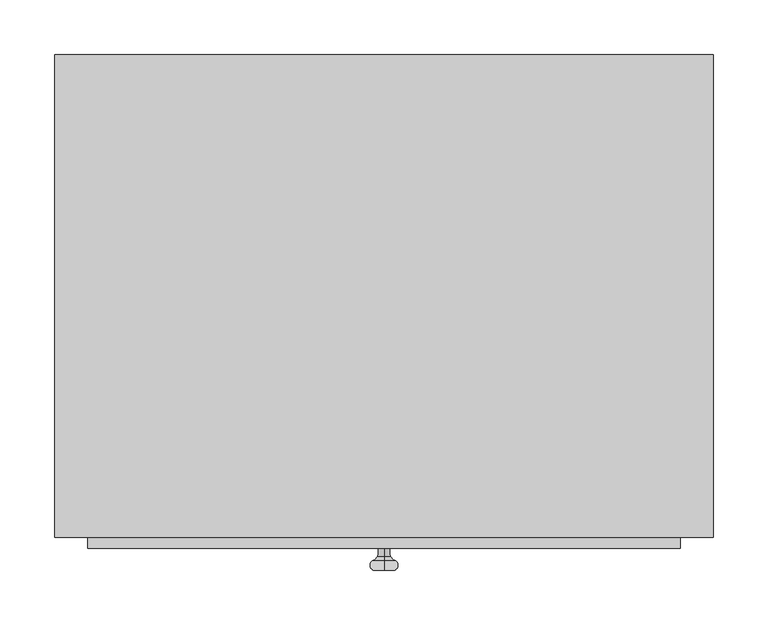
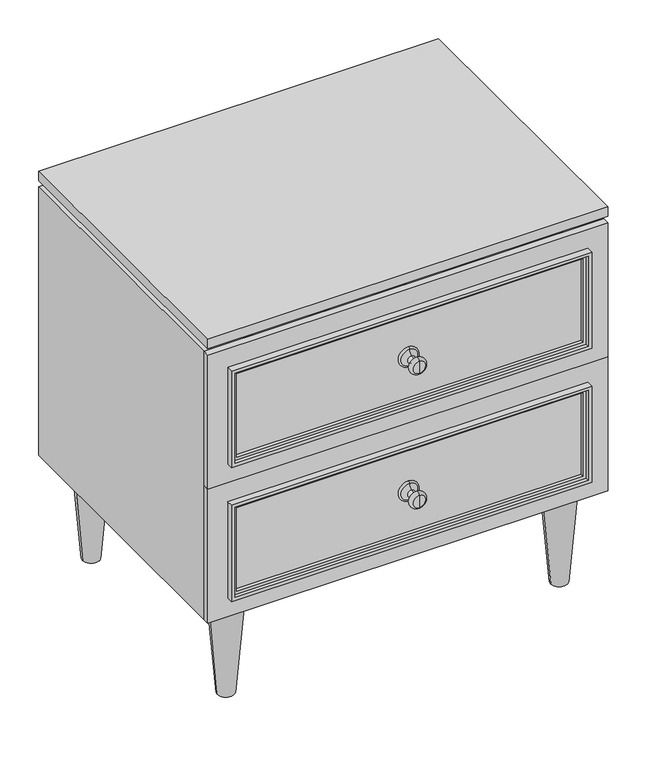
"""IFC4 building model written with IfcOpenShell, lengths in millimetres: proxy geometry, Criado Mudo 02 : Criado Mudo 02."""

from ifc_helpers import new_model, si_unit, point, frame, origin, place, context, project, spatial, polyline, circle_curve, ellipse_curve, trimmed, outline, extrude, faceted_brep, source, transform, mapped, element, save
from ifc_brep_helpers import plane_surface, revolved_surface, advanced_brep


def generic_models_2b41c82f(model_context):
    return source(origin(), model_context, "Body", "SolidModel", [
        advanced_brep(
        [(-237.3303343, 175.0, 0.0), (-262.6696657, 175.0, 0.0), (-225.0, 175.0, 150.0), (-275.0, 175.0, 150.0)],
        [
            (0, 1, circle_curve(frame((-250.0, 175.0, 0.0), z_axis=(0.0, 0.0, -1.0), x_axis=(-1.0, 0.0, 0.0)), 12.6696657)),
            (1, 0, circle_curve(frame((-250.0, 175.0, 0.0), z_axis=(0.0, 0.0, -1.0), x_axis=(1.0, 0.0, 0.0)), 12.6696657)),
            (2, 3, circle_curve(frame((-250.0, 175.0, 150.0), z_axis=(0.0, 0.0, 1.0), x_axis=(1.0, 0.0, 0.0)), 25.0)),
            (3, 2, circle_curve(frame((-250.0, 175.0, 150.0), z_axis=(0.0, 0.0, 1.0), x_axis=(-1.0, 0.0, 0.0)), 25.0)),
            (2, 0),
            (1, 3),
        ],
        [
            plane_surface(frame((-250.0, 175.0, 0.0), z_axis=(0.0, 0.0, -1.0), x_axis=(0.0, -1.0, 0.0))),
            plane_surface(frame((-250.0, 175.0, 150.0), z_axis=(0.0, 0.0, 1.0), x_axis=(0.0, -1.0, 0.0))),
            revolved_surface(polyline([(-237.33033426755935, 175.0, 0.0), (-225.0, 175.0, 150.0)]), (-250.0, 175.0, -154.1280081), (0.0, 0.0, 1.0)),
            revolved_surface(polyline([(-262.66966573244065, 175.0, 0.0), (-275.0, 175.0, 150.0)]), (-250.0, 175.0, -154.1280081), (0.0, 0.0, 1.0)),
        ],
        [
            (0, [[1, 2]]),
            (1, [[3, 4]]),
            (2, [[5, -2, 6, -3]]),
            (3, [[-6, -1, -5, -4]]),
        ],
    ),
        advanced_brep(
        [(237.3303343, 175.0, 0.0), (262.6696657, 175.0, 0.0), (225.0, 175.0, 150.0), (275.0, 175.0, 150.0)],
        [
            (0, 1, circle_curve(frame((250.0, 175.0, 0.0), z_axis=(0.0, 0.0, -1.0), x_axis=(-1.0, 0.0, 0.0)), 12.6696657)),
            (1, 0, circle_curve(frame((250.0, 175.0, 0.0), z_axis=(0.0, 0.0, -1.0), x_axis=(1.0, 0.0, 0.0)), 12.6696657)),
            (2, 3, circle_curve(frame((250.0, 175.0, 150.0), z_axis=(0.0, 0.0, 1.0), x_axis=(1.0, 0.0, 0.0)), 25.0)),
            (3, 2, circle_curve(frame((250.0, 175.0, 150.0), z_axis=(0.0, 0.0, 1.0), x_axis=(-1.0, 0.0, 0.0)), 25.0)),
            (3, 1),
            (0, 2),
        ],
        [
            plane_surface(frame((250.0, 175.0, 0.0), z_axis=(0.0, 0.0, -1.0), x_axis=(0.0, -1.0, 0.0))),
            plane_surface(frame((250.0, 175.0, 150.0), z_axis=(0.0, 0.0, 1.0), x_axis=(0.0, -1.0, 0.0))),
            revolved_surface(polyline([(237.33033426755935, 175.0, 0.0), (225.0, 175.0, 150.0)]), (250.0, 175.0, -154.1280081), (0.0, 0.0, 1.0)),
            revolved_surface(polyline([(262.66966573244065, 175.0, 0.0), (275.0, 175.0, 150.0)]), (250.0, 175.0, -154.1280081), (0.0, 0.0, 1.0)),
        ],
        [
            (0, [[1, 2]]),
            (1, [[3, 4]]),
            (2, [[-4, 5, -1, 6]]),
            (3, [[-3, -6, -2, -5]]),
        ],
    ),
        advanced_brep(
        [(237.3303343, -175.0, 0.0), (262.6696657, -175.0, 0.0), (225.0, -175.0, 150.0), (275.0, -175.0, 150.0)],
        [
            (0, 1, circle_curve(frame((250.0, -175.0, 0.0), z_axis=(0.0, 0.0, -1.0), x_axis=(1.0, 0.0, 0.0)), 12.6696657)),
            (1, 0, circle_curve(frame((250.0, -175.0, 0.0), z_axis=(0.0, 0.0, -1.0), x_axis=(-1.0, 0.0, 0.0)), 12.6696657)),
            (2, 3, circle_curve(frame((250.0, -175.0, 150.0), z_axis=(0.0, 0.0, 1.0), x_axis=(-1.0, 0.0, 0.0)), 25.0)),
            (3, 2, circle_curve(frame((250.0, -175.0, 150.0), z_axis=(0.0, 0.0, 1.0), x_axis=(1.0, 0.0, 0.0)), 25.0)),
            (2, 0),
            (1, 3),
        ],
        [
            plane_surface(frame((250.0, -175.0, 0.0), z_axis=(0.0, 0.0, -1.0), x_axis=(0.0, 1.0, 0.0))),
            plane_surface(frame((250.0, -175.0, 150.0), z_axis=(0.0, 0.0, 1.0), x_axis=(0.0, 1.0, 0.0))),
            revolved_surface(polyline([(237.33033426755935, -175.0, 0.0), (225.0, -175.0, 150.0)]), (250.0, -175.0, -154.1280081), (0.0, 0.0, 1.0)),
            revolved_surface(polyline([(262.66966573244065, -175.0, 0.0), (275.0, -175.0, 150.0)]), (250.0, -175.0, -154.1280081), (0.0, 0.0, 1.0)),
        ],
        [
            (0, [[1, 2]]),
            (1, [[3, 4]]),
            (2, [[5, -2, 6, -3]]),
            (3, [[-6, -1, -5, -4]]),
        ],
    ),
        advanced_brep(
        [(-237.3303343, -175.0, 0.0), (-262.6696657, -175.0, 0.0), (-225.0, -175.0, 150.0), (-275.0, -175.0, 150.0)],
        [
            (0, 1, circle_curve(frame((-250.0, -175.0, 0.0), z_axis=(0.0, 0.0, -1.0), x_axis=(1.0, 0.0, 0.0)), 12.6696657)),
            (1, 0, circle_curve(frame((-250.0, -175.0, 0.0), z_axis=(0.0, 0.0, -1.0), x_axis=(-1.0, 0.0, 0.0)), 12.6696657)),
            (2, 3, circle_curve(frame((-250.0, -175.0, 150.0), z_axis=(0.0, 0.0, 1.0), x_axis=(-1.0, 0.0, 0.0)), 25.0)),
            (3, 2, circle_curve(frame((-250.0, -175.0, 150.0), z_axis=(0.0, 0.0, 1.0), x_axis=(1.0, 0.0, 0.0)), 25.0)),
            (3, 1),
            (0, 2),
        ],
        [
            plane_surface(frame((-250.0, -175.0, 0.0), z_axis=(0.0, 0.0, -1.0), x_axis=(0.0, 1.0, 0.0))),
            plane_surface(frame((-250.0, -175.0, 150.0), z_axis=(0.0, 0.0, 1.0), x_axis=(0.0, 1.0, 0.0))),
            revolved_surface(polyline([(-237.33033426755935, -175.0, 0.0), (-225.0, -175.0, 150.0)]), (-250.0, -175.0, -154.1280081), (0.0, 0.0, 1.0)),
            revolved_surface(polyline([(-262.66966573244065, -175.0, 0.0), (-275.0, -175.0, 150.0)]), (-250.0, -175.0, -154.1280081), (0.0, 0.0, 1.0)),
        ],
        [
            (0, [[1, 2]]),
            (1, [[3, 4]]),
            (2, [[-4, 5, -1, 6]]),
            (3, [[-3, -6, -2, -5]]),
        ],
    ),
        advanced_brep(
        [(0.0, -219.1088234, 455.5505414), (0.0, -219.1088234, 481.9494586), (0.0, -215.0, 481.9494586), (0.0, -215.0, 455.5505414), (0.0, -224.0337931, 462.8521094), (0.0, -224.0337931, 474.6478906), (0.0, -232.2529022, 462.8521094), (0.0, -232.2529022, 474.6478906), (0.0, -236.1458139, 458.9591976), (0.0, -236.1458139, 478.5408024), (0.0, -245.0, 458.9591976), (0.0, -245.0, 478.5408024), (0.0, -245.0, 468.75), (0.0, -215.0, 468.75)],
        [
            (0, 1, circle_curve(frame((0.0, -219.1088234, 468.75), z_axis=(0.0, 1.0, 0.0), x_axis=(0.0, 0.0, 1.0)), 13.1994586)),
            (1, 2, circle_curve(frame((0.0, -217.0544117, 481.9494586), z_axis=(-1.0, 0.0, 0.0), x_axis=(0.0, -1.0, 0.0)), 2.0544117)),
            (2, 3, circle_curve(frame((0.0, -215.0, 468.75), z_axis=(0.0, -1.0, 0.0), x_axis=(0.0, 0.0, 1.0)), 13.1994586)),
            (3, 0, circle_curve(frame((0.0, -217.0544117, 455.5505414), z_axis=(-1.0, 0.0, 0.0), x_axis=(0.0, -1.0, 0.0)), 2.0544117)),
            (1, 0, circle_curve(frame((0.0, -219.1088234, 468.75), z_axis=(0.0, 1.0, 0.0), x_axis=(0.0, 0.0, 1.0)), 13.1994586)),
            (3, 2, circle_curve(frame((0.0, -215.0, 468.75), z_axis=(0.0, -1.0, 0.0), x_axis=(0.0, 0.0, 1.0)), 13.1994586)),
            (4, 5, circle_curve(frame((0.0, -224.0337931, 468.75), z_axis=(0.0, 1.0, 0.0), x_axis=(0.0, 0.0, 1.0)), 5.8978906)),
            (5, 1, circle_curve(frame((0.0, -226.9838181, 481.9494586), z_axis=(1.0, 0.0, 0.0), x_axis=(0.0, -1.0, 0.0)), 7.8749947)),
            (0, 4, circle_curve(frame((0.0, -226.9838181, 455.5505414), z_axis=(1.0, 0.0, 0.0), x_axis=(0.0, -1.0, 0.0)), 7.8749947)),
            (5, 4, circle_curve(frame((0.0, -224.0337931, 468.75), z_axis=(0.0, 1.0, 0.0), x_axis=(0.0, 0.0, 1.0)), 5.8978906)),
            (6, 7, circle_curve(frame((0.0, -232.2529022, 468.75), z_axis=(0.0, 1.0, 0.0), x_axis=(0.0, 0.0, 1.0)), 5.8978906)),
            (7, 5, circle_curve(frame((0.0, -228.1433476, 484.819395), z_axis=(1.0, 0.0, 0.0), x_axis=(0.0, -1.0, 0.0)), 10.9703208)),
            (4, 6, circle_curve(frame((0.0, -228.1433476, 452.680605), z_axis=(1.0, 0.0, 0.0), x_axis=(0.0, -1.0, 0.0)), 10.9703208)),
            (7, 6, circle_curve(frame((0.0, -232.2529022, 468.75), z_axis=(0.0, 1.0, 0.0), x_axis=(0.0, 0.0, 1.0)), 5.8978906)),
            (8, 9, circle_curve(frame((0.0, -236.1458139, 468.75), z_axis=(0.0, 1.0, 0.0), x_axis=(0.0, 0.0, 1.0)), 9.7908024)),
            (9, 7, circle_curve(frame((0.0, -229.6137954, 481.1799091), z_axis=(1.0, 0.0, 0.0), x_axis=(0.0, -1.0, 0.0)), 7.0450089)),
            (6, 8, circle_curve(frame((0.0, -229.6137954, 456.3200909), z_axis=(1.0, 0.0, 0.0), x_axis=(0.0, -1.0, 0.0)), 7.0450089)),
            (9, 8, circle_curve(frame((0.0, -236.1458139, 468.75), z_axis=(0.0, 1.0, 0.0), x_axis=(0.0, 0.0, 1.0)), 9.7908024)),
            (10, 11, circle_curve(frame((0.0, -245.0, 468.75), z_axis=(0.0, 1.0, 0.0), x_axis=(0.0, 0.0, 1.0)), 9.7908024)),
            (11, 9, circle_curve(frame((0.0, -240.5729069, 476.7521407), z_axis=(-1.0, 0.0, 0.0), x_axis=(0.0, -1.0, 0.0)), 4.7747737)),
            (8, 10, circle_curve(frame((0.0, -240.5729069, 460.7478593), z_axis=(-1.0, 0.0, 0.0), x_axis=(0.0, -1.0, 0.0)), 4.7747737)),
            (11, 10, circle_curve(frame((0.0, -245.0, 468.75), z_axis=(0.0, 1.0, 0.0), x_axis=(0.0, 0.0, 1.0)), 9.7908024)),
            (12, 11),
            (10, 12),
            (2, 13),
            (13, 3),
        ],
        [
            revolved_surface(trimmed(ellipse_curve(frame((0.0, -217.0544117, 481.9494586), z_axis=(1.0, 0.0, 0.0), x_axis=(0.0, -1.0, 0.0)), 2.0544117, 2.0544117), [point((0.0, -215.0, 481.9494586))], [point((0.0, -219.1088234, 481.9494586))], True, "CARTESIAN"), (0.0, -215.0, 468.75), (0.0, -1.0, 0.0)),
            revolved_surface(trimmed(ellipse_curve(frame((0.0, -226.9838181, 481.9494586), z_axis=(-1.0, 0.0, 0.0), x_axis=(0.0, -1.0, 0.0)), 7.8749947, 7.8749947), [point((0.0, -219.1088234, 481.9494586))], [point((0.0, -224.0337931, 474.6478906))], True, "CARTESIAN"), (0.0, -215.0, 468.75), (0.0, -1.0, 0.0)),
            revolved_surface(trimmed(ellipse_curve(frame((0.0, -228.1433476, 484.819395), z_axis=(-1.0, 0.0, 0.0), x_axis=(0.0, -1.0, 0.0)), 10.9703208, 10.9703208), [point((0.0, -224.0337931, 474.6478906))], [point((0.0, -232.2529022, 474.6478906))], True, "CARTESIAN"), (0.0, -215.0, 468.75), (0.0, -1.0, 0.0)),
            revolved_surface(trimmed(ellipse_curve(frame((0.0, -229.6137954, 481.1799091), z_axis=(-1.0, 0.0, 0.0), x_axis=(0.0, -1.0, 0.0)), 7.0450089, 7.0450089), [point((0.0, -232.2529022, 474.6478906))], [point((0.0, -236.1458139, 478.5408024))], True, "CARTESIAN"), (0.0, -215.0, 468.75), (0.0, -1.0, 0.0)),
            revolved_surface(trimmed(ellipse_curve(frame((0.0, -240.5729069, 476.7521407), z_axis=(1.0, 0.0, 0.0), x_axis=(0.0, -1.0, 0.0)), 4.7747737, 4.7747737), [point((0.0, -236.1458139, 478.5408024))], [point((0.0, -245.0, 478.5408024))], True, "CARTESIAN"), (0.0, -215.0, 468.75), (0.0, -1.0, 0.0)),
            plane_surface(frame((0.0, -245.0, 468.75), z_axis=(0.0, -1.0, 0.0), x_axis=(0.0, 0.0, 1.0))),
            plane_surface(frame((0.0, -215.0, 468.75), z_axis=(0.0, 1.0, 0.0), x_axis=(0.0, 0.0, 1.0))),
        ],
        [
            (0, [[1, 2, 3, 4]]),
            (0, [[5, -4, 6, -2]]),
            (1, [[7, 8, -1, 9]]),
            (1, [[10, -9, -5, -8]]),
            (2, [[11, 12, -7, 13]]),
            (2, [[14, -13, -10, -12]]),
            (3, [[15, 16, -11, 17]]),
            (3, [[18, -17, -14, -16]]),
            (4, [[19, 20, -15, 21]]),
            (4, [[22, -21, -18, -20]]),
            (5, [[23, -19, 24]]),
            (5, [[-24, -22, -23]]),
            (6, [[-3, 25, 26]]),
            (6, [[-6, -26, -25]]),
        ],
    ),
        faceted_brep([(270.0, -215.0, 545.0), (270.0, -225.0, 545.0), (270.0, -225.0, 392.5), (270.0, -215.0, 392.5), (260.0, -220.0, 535.0), (260.0, -215.0, 535.0), (260.0, -215.0, 402.5), (260.0, -220.0, 402.5), (265.0, -225.0, 540.0), (265.0, -220.0, 540.0), (265.0, -220.0, 397.5), (265.0, -225.0, 397.5), (-270.0, -225.0, 392.5), (-270.0, -215.0, 392.5), (-260.0, -215.0, 402.5), (-260.0, -220.0, 402.5), (-265.0, -220.0, 397.5), (-265.0, -225.0, 397.5), (-270.0, -225.0, 545.0), (-270.0, -215.0, 545.0), (-260.0, -215.0, 535.0), (-260.0, -220.0, 535.0), (-265.0, -220.0, 540.0), (-265.0, -225.0, 540.0)], [[[0, 1, 2, 3]], [[4, 5, 6, 7]], [[8, 9, 10, 11]], [[3, 2, 12, 13]], [[7, 6, 14, 15]], [[11, 10, 16, 17]], [[13, 12, 18, 19]], [[15, 14, 20, 21]], [[17, 16, 22, 23]], [[19, 18, 1, 0]], [[3, 13, 19, 0], [5, 20, 14, 6]], [[21, 20, 5, 4]], [[9, 22, 16, 10], [7, 15, 21, 4]], [[23, 22, 9, 8]], [[1, 18, 12, 2], [11, 17, 23, 8]]]),
        extrude(outline(polyline([(300.0, -215.0), (-300.0, -215.0), (-300.0, -205.0), (300.0, -205.0), (300.0, -215.0)])), frame((0.0, 0.0, 362.5), z_axis=(0.0, 0.0, 1.0), x_axis=(1.0, 0.0, 0.0)), (0.0, 0.0, 1.0), 212.5),
        extrude(outline(polyline([(277.5, -205.0), (-277.5, -205.0), (-277.5, 200.0), (277.5, 200.0), (277.5, -205.0)])), frame((0.0, 0.0, 392.5), z_axis=(0.0, 0.0, 1.0), x_axis=(1.0, 0.0, 0.0)), (0.0, 0.0, 1.0), 15.0),
        extrude(outline(polyline([(262.5, 200.0), (262.5, 185.0), (-262.5, 185.0), (-262.5, 200.0), (262.5, 200.0)])), frame((0.0, 0.0, 407.5), z_axis=(0.0, 0.0, 1.0), x_axis=(1.0, 0.0, 0.0)), (0.0, 0.0, 1.0), 137.5),
        extrude(outline(polyline([(262.5, 200.0), (277.5, 200.0), (277.5, -205.0), (262.5, -205.0), (262.5, 200.0)])), frame((0.0, 0.0, 407.5), z_axis=(0.0, 0.0, 1.0), x_axis=(1.0, 0.0, 0.0)), (0.0, 0.0, 1.0), 137.5),
        extrude(outline(polyline([(-262.5, 200.0), (-262.5, -205.0), (-277.5, -205.0), (-277.5, 200.0), (-262.5, 200.0)])), frame((0.0, 0.0, 407.5), z_axis=(0.0, 0.0, 1.0), x_axis=(1.0, 0.0, 0.0)), (0.0, 0.0, 1.0), 137.5),
        advanced_brep(
        [(0.0, -219.1088234, 243.0505414), (0.0, -219.1088234, 269.4494586), (0.0, -215.0, 269.4494586), (0.0, -215.0, 243.0505414), (0.0, -224.0337931, 250.3521094), (0.0, -224.0337931, 262.1478906), (0.0, -232.2529022, 250.3521094), (0.0, -232.2529022, 262.1478906), (0.0, -236.1458139, 246.4591976), (0.0, -236.1458139, 266.0408024), (0.0, -245.0, 246.4591976), (0.0, -245.0, 266.0408024), (0.0, -245.0, 256.25), (0.0, -215.0, 256.25)],
        [
            (0, 1, circle_curve(frame((0.0, -219.1088234, 256.25), z_axis=(0.0, 1.0, 0.0), x_axis=(0.0, 0.0, 1.0)), 13.1994586)),
            (1, 2, circle_curve(frame((0.0, -217.0544117, 269.4494586), z_axis=(-1.0, 0.0, 0.0), x_axis=(0.0, -1.0, 0.0)), 2.0544117)),
            (2, 3, circle_curve(frame((0.0, -215.0, 256.25), z_axis=(0.0, -1.0, 0.0), x_axis=(0.0, 0.0, 1.0)), 13.1994586)),
            (3, 0, circle_curve(frame((0.0, -217.0544117, 243.0505414), z_axis=(-1.0, 0.0, 0.0), x_axis=(0.0, -1.0, 0.0)), 2.0544117)),
            (1, 0, circle_curve(frame((0.0, -219.1088234, 256.25), z_axis=(0.0, 1.0, 0.0), x_axis=(0.0, 0.0, 1.0)), 13.1994586)),
            (3, 2, circle_curve(frame((0.0, -215.0, 256.25), z_axis=(0.0, -1.0, 0.0), x_axis=(0.0, 0.0, 1.0)), 13.1994586)),
            (4, 5, circle_curve(frame((0.0, -224.0337931, 256.25), z_axis=(0.0, 1.0, 0.0), x_axis=(0.0, 0.0, 1.0)), 5.8978906)),
            (5, 1, circle_curve(frame((0.0, -226.9838181, 269.4494586), z_axis=(1.0, 0.0, 0.0), x_axis=(0.0, -1.0, 0.0)), 7.8749947)),
            (0, 4, circle_curve(frame((0.0, -226.9838181, 243.0505414), z_axis=(1.0, 0.0, 0.0), x_axis=(0.0, -1.0, 0.0)), 7.8749947)),
            (5, 4, circle_curve(frame((0.0, -224.0337931, 256.25), z_axis=(0.0, 1.0, 0.0), x_axis=(0.0, 0.0, 1.0)), 5.8978906)),
            (6, 7, circle_curve(frame((0.0, -232.2529022, 256.25), z_axis=(0.0, 1.0, 0.0), x_axis=(0.0, 0.0, 1.0)), 5.8978906)),
            (7, 5, circle_curve(frame((0.0, -228.1433476, 272.319395), z_axis=(1.0, 0.0, 0.0), x_axis=(0.0, -1.0, 0.0)), 10.9703208)),
            (4, 6, circle_curve(frame((0.0, -228.1433476, 240.180605), z_axis=(1.0, 0.0, 0.0), x_axis=(0.0, -1.0, 0.0)), 10.9703208)),
            (7, 6, circle_curve(frame((0.0, -232.2529022, 256.25), z_axis=(0.0, 1.0, 0.0), x_axis=(0.0, 0.0, 1.0)), 5.8978906)),
            (8, 9, circle_curve(frame((0.0, -236.1458139, 256.25), z_axis=(0.0, 1.0, 0.0), x_axis=(0.0, 0.0, 1.0)), 9.7908024)),
            (9, 7, circle_curve(frame((0.0, -229.6137954, 268.6799091), z_axis=(1.0, 0.0, 0.0), x_axis=(0.0, -1.0, 0.0)), 7.0450089)),
            (6, 8, circle_curve(frame((0.0, -229.6137954, 243.8200909), z_axis=(1.0, 0.0, 0.0), x_axis=(0.0, -1.0, 0.0)), 7.0450089)),
            (9, 8, circle_curve(frame((0.0, -236.1458139, 256.25), z_axis=(0.0, 1.0, 0.0), x_axis=(0.0, 0.0, 1.0)), 9.7908024)),
            (10, 11, circle_curve(frame((0.0, -245.0, 256.25), z_axis=(0.0, 1.0, 0.0), x_axis=(0.0, 0.0, 1.0)), 9.7908024)),
            (11, 9, circle_curve(frame((0.0, -240.5729069, 264.2521407), z_axis=(-1.0, 0.0, 0.0), x_axis=(0.0, -1.0, 0.0)), 4.7747737)),
            (8, 10, circle_curve(frame((0.0, -240.5729069, 248.2478593), z_axis=(-1.0, 0.0, 0.0), x_axis=(0.0, -1.0, 0.0)), 4.7747737)),
            (11, 10, circle_curve(frame((0.0, -245.0, 256.25), z_axis=(0.0, 1.0, 0.0), x_axis=(0.0, 0.0, 1.0)), 9.7908024)),
            (12, 11),
            (10, 12),
            (2, 13),
            (13, 3),
        ],
        [
            revolved_surface(trimmed(ellipse_curve(frame((0.0, -217.0544117, 269.4494586), z_axis=(1.0, 0.0, 0.0), x_axis=(0.0, -1.0, 0.0)), 2.0544117, 2.0544117), [point((0.0, -215.0, 269.4494586))], [point((0.0, -219.1088234, 269.4494586))], True, "CARTESIAN"), (0.0, -215.0, 256.25), (0.0, -1.0, 0.0)),
            revolved_surface(trimmed(ellipse_curve(frame((0.0, -226.9838181, 269.4494586), z_axis=(-1.0, 0.0, 0.0), x_axis=(0.0, -1.0, 0.0)), 7.8749947, 7.8749947), [point((0.0, -219.1088234, 269.4494586))], [point((0.0, -224.0337931, 262.1478906))], True, "CARTESIAN"), (0.0, -215.0, 256.25), (0.0, -1.0, 0.0)),
            revolved_surface(trimmed(ellipse_curve(frame((0.0, -228.1433476, 272.319395), z_axis=(-1.0, 0.0, 0.0), x_axis=(0.0, -1.0, 0.0)), 10.9703208, 10.9703208), [point((0.0, -224.0337931, 262.1478906))], [point((0.0, -232.2529022, 262.1478906))], True, "CARTESIAN"), (0.0, -215.0, 256.25), (0.0, -1.0, 0.0)),
            revolved_surface(trimmed(ellipse_curve(frame((0.0, -229.6137954, 268.6799091), z_axis=(-1.0, 0.0, 0.0), x_axis=(0.0, -1.0, 0.0)), 7.0450089, 7.0450089), [point((0.0, -232.2529022, 262.1478906))], [point((0.0, -236.1458139, 266.0408024))], True, "CARTESIAN"), (0.0, -215.0, 256.25), (0.0, -1.0, 0.0)),
            revolved_surface(trimmed(ellipse_curve(frame((0.0, -240.5729069, 264.2521407), z_axis=(1.0, 0.0, 0.0), x_axis=(0.0, -1.0, 0.0)), 4.7747737, 4.7747737), [point((0.0, -236.1458139, 266.0408024))], [point((0.0, -245.0, 266.0408024))], True, "CARTESIAN"), (0.0, -215.0, 256.25), (0.0, -1.0, 0.0)),
            plane_surface(frame((0.0, -245.0, 256.25), z_axis=(0.0, -1.0, 0.0), x_axis=(0.0, 0.0, 1.0))),
            plane_surface(frame((0.0, -215.0, 256.25), z_axis=(0.0, 1.0, 0.0), x_axis=(0.0, 0.0, 1.0))),
        ],
        [
            (0, [[1, 2, 3, 4]]),
            (0, [[5, -4, 6, -2]]),
            (1, [[7, 8, -1, 9]]),
            (1, [[10, -9, -5, -8]]),
            (2, [[11, 12, -7, 13]]),
            (2, [[14, -13, -10, -12]]),
            (3, [[15, 16, -11, 17]]),
            (3, [[18, -17, -14, -16]]),
            (4, [[19, 20, -15, 21]]),
            (4, [[22, -21, -18, -20]]),
            (5, [[23, -19, 24]]),
            (5, [[-24, -22, -23]]),
            (6, [[-3, 25, 26]]),
            (6, [[-6, -26, -25]]),
        ],
    ),
        faceted_brep([(270.0, -215.0, 332.5), (270.0, -225.0, 332.5), (270.0, -225.0, 180.0), (270.0, -215.0, 180.0), (260.0, -220.0, 322.5), (260.0, -215.0, 322.5), (260.0, -215.0, 190.0), (260.0, -220.0, 190.0), (265.0, -225.0, 327.5), (265.0, -220.0, 327.5), (265.0, -220.0, 185.0), (265.0, -225.0, 185.0), (-270.0, -225.0, 180.0), (-270.0, -215.0, 180.0), (-260.0, -215.0, 190.0), (-260.0, -220.0, 190.0), (-265.0, -220.0, 185.0), (-265.0, -225.0, 185.0), (-270.0, -225.0, 332.5), (-270.0, -215.0, 332.5), (-260.0, -215.0, 322.5), (-260.0, -220.0, 322.5), (-265.0, -220.0, 327.5), (-265.0, -225.0, 327.5)], [[[0, 1, 2, 3]], [[4, 5, 6, 7]], [[8, 9, 10, 11]], [[3, 2, 12, 13]], [[7, 6, 14, 15]], [[11, 10, 16, 17]], [[13, 12, 18, 19]], [[15, 14, 20, 21]], [[17, 16, 22, 23]], [[19, 18, 1, 0]], [[3, 13, 19, 0], [5, 20, 14, 6]], [[21, 20, 5, 4]], [[9, 22, 16, 10], [7, 15, 21, 4]], [[23, 22, 9, 8]], [[1, 18, 12, 2], [11, 17, 23, 8]]]),
        extrude(outline(polyline([(300.0, -215.0), (-300.0, -215.0), (-300.0, -205.0), (300.0, -205.0), (300.0, -215.0)])), frame((0.0, 0.0, 150.0), z_axis=(0.0, 0.0, 1.0), x_axis=(1.0, 0.0, 0.0)), (0.0, 0.0, 1.0), 212.5),
        extrude(outline(polyline([(277.5, -205.0), (-277.5, -205.0), (-277.5, 200.0), (277.5, 200.0), (277.5, -205.0)])), frame((0.0, 0.0, 180.0), z_axis=(0.0, 0.0, 1.0), x_axis=(1.0, 0.0, 0.0)), (0.0, 0.0, 1.0), 15.0),
        extrude(outline(polyline([(262.5, 200.0), (262.5, 185.0), (-262.5, 185.0), (-262.5, 200.0), (262.5, 200.0)])), frame((0.0, 0.0, 195.0), z_axis=(0.0, 0.0, 1.0), x_axis=(1.0, 0.0, 0.0)), (0.0, 0.0, 1.0), 137.5),
        extrude(outline(polyline([(262.5, 200.0), (277.5, 200.0), (277.5, -205.0), (262.5, -205.0), (262.5, 200.0)])), frame((0.0, 0.0, 195.0), z_axis=(0.0, 0.0, 1.0), x_axis=(1.0, 0.0, 0.0)), (0.0, 0.0, 1.0), 137.5),
        extrude(outline(polyline([(-262.5, 200.0), (-262.5, -205.0), (-277.5, -205.0), (-277.5, 200.0), (-262.5, 200.0)])), frame((0.0, 0.0, 195.0), z_axis=(0.0, 0.0, 1.0), x_axis=(1.0, 0.0, 0.0)), (0.0, 0.0, 1.0), 137.5),
        faceted_brep([(300.0, -205.0, 150.0), (300.0, -205.0, 575.0), (-300.0, -205.0, 575.0), (-300.0, -205.0, 150.0), (285.0, -205.0, 165.0), (-285.0, -205.0, 165.0), (-285.0, -205.0, 560.0), (285.0, -205.0, 560.0), (300.0, 225.0, 150.0), (-300.0, 225.0, 150.0), (-300.0, 225.0, 575.0), (300.0, 225.0, 575.0), (285.0, 210.0, 560.0), (285.0, 210.0, 165.0), (-285.0, 210.0, 165.0), (-285.0, 210.0, 560.0)], [[[0, 1, 2, 3], [4, 5, 6, 7]], [[8, 9, 10, 11]], [[1, 0, 8, 11]], [[11, 10, 2, 1]], [[4, 7, 12, 13]], [[5, 4, 13, 14]], [[6, 5, 14, 15]], [[3, 2, 10, 9]], [[0, 3, 9, 8]], [[7, 6, 15, 12]], [[13, 12, 15, 14]]]),
        faceted_brep([(290.0, -205.0, 585.0), (290.0, -205.0, 575.0), (290.0, 215.0, 575.0), (290.0, 215.0, 585.0), (300.0, -215.0, 600.0), (300.0, -215.0, 585.0), (300.0, 225.0, 585.0), (300.0, 225.0, 600.0), (-290.0, 215.0, 575.0), (-290.0, 215.0, 585.0), (-300.0, 225.0, 585.0), (-300.0, 225.0, 600.0), (-290.0, -205.0, 575.0), (-290.0, -205.0, 585.0), (-300.0, -215.0, 585.0), (-300.0, -215.0, 600.0)], [[[0, 1, 2, 3]], [[4, 5, 6, 7]], [[3, 2, 8, 9]], [[7, 6, 10, 11]], [[9, 8, 12, 13]], [[11, 10, 14, 15]], [[2, 1, 12, 8]], [[1, 0, 13, 12]], [[6, 5, 14, 10], [0, 3, 9, 13]], [[5, 4, 15, 14]], [[4, 7, 11, 15]]]),
    ])


if __name__ == "__main__":
    model = new_model("IFC4")
    model_context = context("Model", 3, world=origin())
    ifc_project = project(units=[si_unit("LENGTHUNIT", "METRE", prefix="MILLI")], contexts=[model_context])
    site = spatial("IfcSite", under=ifc_project)
    building = spatial("IfcBuilding", under=site)
    placement = place(None, origin())
    generic_models_shape = generic_models_2b41c82f(model_context)
    element("IfcBuildingElementProxy", 1, Name="Criado Mudo 02 : Criado Mudo 02", ObjectType="Criado Mudo 02 : Criado Mudo 02", at=placement, inside=building, context=model_context, shape_type="MappedRepresentation", body=[
        mapped(generic_models_shape, transform((0.0, 0.0, 0.0), x_axis=(1.0, 0.0, 0.0), y_axis=(0.0, 1.0, 0.0), z_axis=(0.0, 0.0, 1.0))),
    ])
    save(model, "model.ifc")

# Revit data of these elements
# Type "Criado Mudo 02 : Criado Mudo 02"
#   URL = "www.vitrinerevit.com"
#   Description = "Baixe famílias gratuitas no site!"
#   Profundidade = 450 mm
#   Comprimento = 600 mm
#   Altura = 600 mm
#   Quantidade Gavetas = 2
#   Material Pés = Cherry
#   Material Puxador = Laca Branca
#   Material = Cor 05
# Element 1 (IfcBuildingElementProxy, "Criado Mudo 02 : Criado Mudo 02")
#   Materials on its faces: "Cor 05", "Laca Branca", "Cherry"
# Materials
#   "Cherry": class "Wood", colour RGB 154 107 61, transparency 0, Description = "Prunus Serotina", Cost = 0
#   "Laca Branca": class "Generic", colour RGB 255 255 255, transparency 0, Cost = 0
#   "Cor 05": class "Generic", colour RGB 162 153 138, transparency 0, Cost = 0
